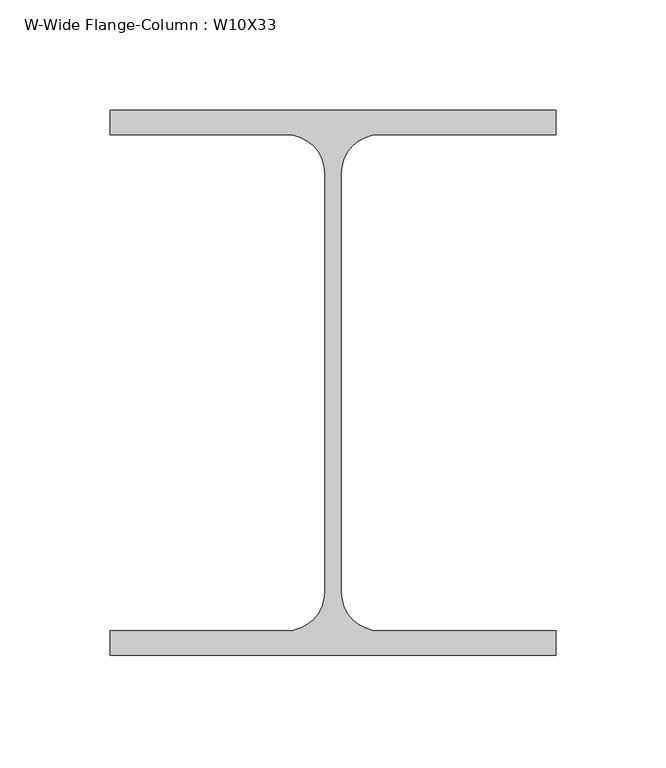
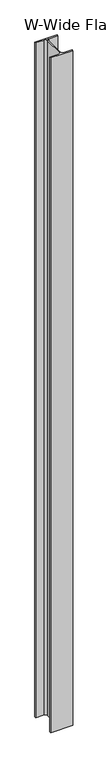
"""IFC4 building model written with IfcOpenShell, lengths in millimetres: column geometry, W-Wide Flange-Column : W10X33."""

import ifcopenshell
import ifcopenshell.guid

model = None  # the IFC model being written
_history = None  # IfcOwnerHistory: only IFC2X3 demands one
_inside = {}  # id of a spatial element -> (the spatial element, [elements in it])
_under = {}  # id of a project, library or spatial element -> (it, [spatial elements below it])
_declared = {}  # id of a project -> (the project, [libraries it declares])
_typed = {}  # id of a type object -> (the type object, [elements of that type])
_made_of = {}  # id of a material, layer set ... -> (it, [elements and type objects made of it])


def new_model(schema):
    """Start an empty IFC model of exactly this schema.

    Asked for "IFC4X3", IfcOpenShell would pick the latest addendum, in which some entities
    have other attributes; the version numbers below select the first issue.
    IFC2X3 requires an IfcOwnerHistory on every rooted entity: one is made here for all.
    """
    global model, _history
    if schema == "IFC4X3":
        model = ifcopenshell.file(schema_version=(4, 3, 0, 0))
    else:
        model = ifcopenshell.file(schema=schema)
    _inside.clear()
    _under.clear()
    _declared.clear()
    _typed.clear()
    _made_of.clear()
    _history = None
    if model.schema == "IFC2X3":
        org = make("IfcOrganization", Name="unknown")
        user = make(
            "IfcPersonAndOrganization",
            ThePerson=make("IfcPerson", FamilyName="unknown"),
            TheOrganization=org,
        )
        app = make(
            "IfcApplication",
            ApplicationDeveloper=org,
            Version="unknown",
            ApplicationFullName="unknown",
            ApplicationIdentifier="unknown",
        )
        _history = make(
            "IfcOwnerHistory",
            OwningUser=user,
            OwningApplication=app,
            ChangeAction="ADDED",
            CreationDate=0,
        )
    return model


def make(cls, **values):
    """One entity of the class cls with the attributes given. An attribute that is None is left unset."""
    return model.create_entity(
        cls, **{name: value for name, value in values.items() if value is not None}
    )


def rooted(cls, **values):
    """An entity with a GlobalId (a new one), such as an element, a storey or a relation."""
    return make(cls, GlobalId=ifcopenshell.guid.new(), OwnerHistory=_history, **values)


def si_unit(unit_type, name, prefix=None):
    """IfcSIUnit, for example si_unit("LENGTHUNIT", "METRE", prefix="MILLI")."""
    return make("IfcSIUnit", UnitType=unit_type, Prefix=prefix, Name=name)


def assignment(units):
    """IfcUnitAssignment: the units of a project."""
    return None if units is None else make("IfcUnitAssignment", Units=units)


def point(xyz):
    """IfcCartesianPoint."""
    return None if xyz is None else make("IfcCartesianPoint", Coordinates=xyz)


def direction(xyz):
    """IfcDirection."""
    return None if xyz is None else make("IfcDirection", DirectionRatios=xyz)


def frame(location, z_axis=None, x_axis=None):
    """IfcAxis2Placement3D, a coordinate frame: its origin and axes. An axis left out is left unset."""
    return make(
        "IfcAxis2Placement3D",
        Location=point(location),
        Axis=direction(z_axis),
        RefDirection=direction(x_axis),
    )


def frame_2d(location, x_axis=None):
    """IfcAxis2Placement2D, a coordinate frame in the plane: its origin and x axis."""
    return make(
        "IfcAxis2Placement2D", Location=point(location), RefDirection=direction(x_axis)
    )


def origin():
    """The frame at (0, 0, 0) with its axes left unset."""
    return frame((0.0, 0.0, 0.0))


def place(relative_to, where):
    """IfcLocalPlacement: puts the frame where relative to a parent placement (None: the world)."""
    return make(
        "IfcLocalPlacement", PlacementRelTo=relative_to, RelativePlacement=where
    )


def context(
    kind, dimensions, precision=None, world=None, true_north=None, identifier=None
):
    """IfcGeometricRepresentationContext, for example the 3D "Model" context."""
    return make(
        "IfcGeometricRepresentationContext",
        ContextIdentifier=identifier,
        ContextType=kind,
        CoordinateSpaceDimension=dimensions,
        Precision=precision,
        WorldCoordinateSystem=world,
        TrueNorth=true_north,
    )


def project(units=None, contexts=None):
    """IfcProject with its units and contexts."""
    return rooted(
        "IfcProject",
        Name="project",
        RepresentationContexts=contexts,
        UnitsInContext=assignment(units),
    )


def spatial(cls, under=None, at=None, **own):
    """A site, building, storey or space (cls), placed at a placement, below another one or the project."""
    s = rooted(cls, ObjectPlacement=at, **own)
    if under is not None:
        _under.setdefault(under.id(), (under, []))[1].append(s)
    return s


def polyline(points):
    """IfcPolyline through the points."""
    return make("IfcPolyline", Points=[point(p) for p in points])


def circle_curve(where, radius):
    """IfcCircle in the frame where."""
    return make("IfcCircle", Position=where, Radius=radius)


def trimmed(basis, trim1, trim2, sense, master):
    """IfcTrimmedCurve: the piece of a basis curve between two trims."""
    return make(
        "IfcTrimmedCurve",
        BasisCurve=basis,
        Trim1=trim1,
        Trim2=trim2,
        SenseAgreement=sense,
        MasterRepresentation=master,
    )


def segment(curve, same_sense, transition):
    """IfcCompositeCurveSegment."""
    return make(
        "IfcCompositeCurveSegment",
        Transition=transition,
        SameSense=same_sense,
        ParentCurve=curve,
    )


def composite_curve(segments, self_intersect=None):
    """IfcCompositeCurve: segments joined end to end."""
    return make("IfcCompositeCurve", Segments=segments, SelfIntersect=self_intersect)


def outline(outer, holes=None, kind="AREA"):
    """IfcArbitraryClosedProfileDef: a profile drawn as a closed curve; with holes, ...WithVoids."""
    if holes is None:
        return make("IfcArbitraryClosedProfileDef", ProfileType=kind, OuterCurve=outer)
    return make(
        "IfcArbitraryProfileDefWithVoids",
        ProfileType=kind,
        OuterCurve=outer,
        InnerCurves=holes,
    )


def extrude(swept, where, along, depth):
    """IfcExtrudedAreaSolid: the profile swept, set in the frame where, extruded along a direction by depth."""
    return make(
        "IfcExtrudedAreaSolid",
        SweptArea=swept,
        Position=where,
        ExtrudedDirection=direction(along),
        Depth=depth,
    )


def shape(context_of_items, identifier, shape_type, items):
    """IfcShapeRepresentation: the items that make up one representation, for example the "Body"."""
    return make(
        "IfcShapeRepresentation",
        ContextOfItems=context_of_items,
        RepresentationIdentifier=identifier,
        RepresentationType=shape_type,
        Items=items,
    )


def source(mapping_origin, context_of_items, identifier, shape_type, items):
    """IfcRepresentationMap: a shape defined once, which mapped items show again and again."""
    return make(
        "IfcRepresentationMap",
        MappingOrigin=mapping_origin,
        MappedRepresentation=shape(context_of_items, identifier, shape_type, items),
    )


def transform(
    local_origin,
    x_axis=None,
    y_axis=None,
    z_axis=None,
    scale=None,
    scale2=None,
    scale3=None,
    uniform=True,
):
    """IfcCartesianTransformationOperator3D, or its non-uniform kind. x_axis, y_axis, z_axis: its Axis1, 2, 3."""
    if uniform:
        return make(
            "IfcCartesianTransformationOperator3D",
            Axis1=direction(x_axis),
            Axis2=direction(y_axis),
            LocalOrigin=point(local_origin),
            Scale=scale,
            Axis3=direction(z_axis),
        )
    return make(
        "IfcCartesianTransformationOperator3DnonUniform",
        Axis1=direction(x_axis),
        Axis2=direction(y_axis),
        LocalOrigin=point(local_origin),
        Scale=scale,
        Axis3=direction(z_axis),
        Scale2=scale2,
        Scale3=scale3,
    )


def mapped(mapping_source, mapping_target):
    """IfcMappedItem: shows the shape of a source again, moved by a transform."""
    return make(
        "IfcMappedItem", MappingSource=mapping_source, MappingTarget=mapping_target
    )


def made_of(thing, what):
    """Note that an element or type object is made of a material, layer set ...; save() writes the relation."""
    if what is not None:
        _made_of.setdefault(what.id(), (what, []))[1].append(thing)
    return thing


def element(
    cls,
    number,
    at=None,
    inside=None,
    cuts=None,
    type_object=None,
    material=None,
    context=None,
    identifier="Body",
    shape_type=None,
    held_by="IfcProductDefinitionShape",
    body=None,
    shapes=None,
    **own,
):
    """One element of the class cls, such as IfcWall. Its Tag is "e" and its number.

    at: its placement. inside: the storey or other place that contains it. cuts: it is an
    opening in that element (IfcRelVoidsElement). A single representation is given by context,
    identifier, shape_type and body (its items); several are given by shapes. held_by: the class
    of the entity that holds the representations. save() writes the other relations.
    """
    e = rooted(cls, Tag="e%d" % number, ObjectPlacement=at, **own)
    if body is not None:
        shapes = [shape(context, identifier, shape_type, body)]
    if shapes is not None:
        e.Representation = make(held_by, Representations=shapes)
    if inside is not None:
        _inside.setdefault(inside.id(), (inside, []))[1].append(e)
    if cuts is not None:
        rooted(
            "IfcRelVoidsElement", RelatingBuildingElement=cuts, RelatedOpeningElement=e
        )
    if type_object is not None:
        _typed.setdefault(type_object.id(), (type_object, []))[1].append(e)
    return made_of(e, material)


def aggregate(whole, parts):
    """IfcRelAggregates: a whole, such as a stair, and the parts it consists of."""
    return rooted("IfcRelAggregates", RelatingObject=whole, RelatedObjects=parts)


def save(model, path):
    """Write the relations noted so far, then the file.

    IfcRelAggregates (storeys below a building ...), IfcRelContainedInSpatialStructure (elements
    in a storey), IfcRelDefinesByType, IfcRelAssociatesMaterial and IfcRelDeclares: one each for
    every whole, place, type object, material and project.
    """
    for whole, parts in _under.values():
        aggregate(whole, parts)
    for where, things in _inside.values():
        rooted(
            "IfcRelContainedInSpatialStructure",
            RelatedElements=things,
            RelatingStructure=where,
        )
    for kind, things in _typed.values():
        rooted("IfcRelDefinesByType", RelatedObjects=things, RelatingType=kind)
    for what, things in _made_of.values():
        rooted("IfcRelAssociatesMaterial", RelatedObjects=things, RelatingMaterial=what)
    for by, libraries in _declared.values():
        rooted("IfcRelDeclares", RelatingContext=by, RelatedDefinitions=libraries)
    model.write(path)


def w_wide_flange_column_w10x33_69d6c3d7(model_context):
    return source(origin(), model_context, "Body", "SweptSolid", [
        extrude(outline(composite_curve([segment(polyline([(101.092, 123.571), (101.092, 112.522), (21.209, 112.522)]), True, "CONTINUOUS"), segment(trimmed(circle_curve(frame_2d((21.209, 94.996)), 17.526), [point((21.209, 112.522))], [point((3.683, 94.996))], True, "CARTESIAN"), True, "CONTINUOUS"), segment(polyline([(3.683, 94.996), (3.683, -94.996)]), True, "CONTINUOUS"), segment(trimmed(circle_curve(frame_2d((21.209, -94.996)), 17.526), [point((3.683, -94.996))], [point((21.209, -112.522))], True, "CARTESIAN"), True, "CONTINUOUS"), segment(polyline([(21.209, -112.522), (101.092, -112.522), (101.092, -123.571), (-101.092, -123.571), (-101.092, -112.522), (-21.209, -112.522)]), True, "CONTINUOUS"), segment(trimmed(circle_curve(frame_2d((-21.209, -94.996)), 17.526), [point((-21.209, -112.522))], [point((-3.683, -94.996))], True, "CARTESIAN"), True, "CONTINUOUS"), segment(polyline([(-3.683, -94.996), (-3.683, 94.996)]), True, "CONTINUOUS"), segment(trimmed(circle_curve(frame_2d((-21.209, 94.996)), 17.526), [point((-3.683, 94.996))], [point((-21.209, 112.522))], True, "CARTESIAN"), True, "CONTINUOUS"), segment(polyline([(-21.209, 112.522), (-101.092, 112.522), (-101.092, 123.571), (101.092, 123.571)]), True, "CONTINUOUS")], self_intersect=False)), frame((0.0, 0.0, 12566.65), z_axis=(0.0, 0.0, 1.0), x_axis=(1.0, 0.0, 0.0)), (0.0, 0.0, 1.0), 6483.35),
    ])


if __name__ == "__main__":
    model = new_model("IFC4")
    model_context = context("Model", 3, world=origin())
    ifc_project = project(units=[si_unit("LENGTHUNIT", "METRE", prefix="MILLI")], contexts=[model_context])
    site = spatial("IfcSite", under=ifc_project)
    building = spatial("IfcBuilding", under=site)
    placement = place(None, origin())
    w_wide_flange_column_w10x33_shape = w_wide_flange_column_w10x33_69d6c3d7(model_context)
    element("IfcColumn", 1, ObjectType="W-Wide Flange-Column : W10X33", at=placement, inside=building, context=model_context, shape_type="MappedRepresentation", body=[
        mapped(w_wide_flange_column_w10x33_shape, transform((0.0, 0.0, 0.0), x_axis=(1.0, 0.0, 0.0), y_axis=(0.0, 1.0, 0.0), z_axis=(0.0, 0.0, 1.0))),
    ])
    save(model, "model.ifc")

# Revit data of these elements
# Type "W-Wide Flange-Column : W10X33"
#   Assembly Code = "B10"
#   W = 33
#   bf = 0' - 7.96"
#   d = 0' - 9.73"
#   k = 0' - 1 1/8"
#   kr = 0' - 0.69"
#   tf = 0' - 0.435"
#   tw = 0' - 0.29"
#   A = 0.0674306 SF
#   Structural Material [instance default] = Steel ASTM A992
# Element 1 (IfcColumn, "W-Wide Flange-Column : W10X33")
#   Materials on its faces: "Steel ASTM A992"
# Materials
#   "Steel ASTM A992": class "Metal", colour RGB 199 199 199, transparency 0, Description = "Structural steel 50ksi", Cost = 0
